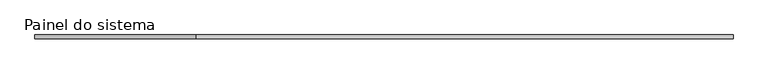
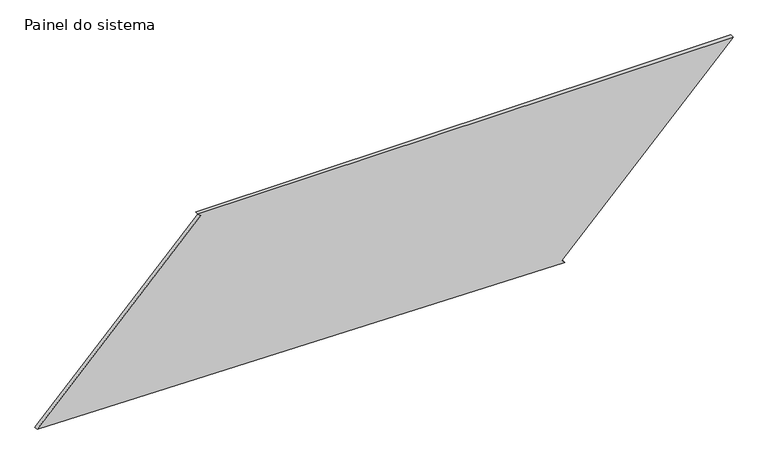
"""IFC4 building model written with IfcOpenShell, lengths in millimetres: plate geometry, Painel do sistema : Envidraçado."""

from ifc_helpers import new_model, si_unit, frame, origin, place, context, project, spatial, polyline, outline, extrude, source, transform, mapped, element, save


def painel_do_sistema_521c3f7b(model_context):
    return source(origin(), model_context, "Body", "SweptSolid", [
        extrude(outline(polyline([(0.0, 1189.455297), (17.3932625, 1171.4977243), (1188.7683803, 2306.0628062), (1188.7683803, -1240.670622), (1171.3751177, -1222.7130493), (52.8769643, -2306.0628062), (0.0, 1189.455297)])), frame((0.0, 24.5, 0.0), z_axis=(0.0, 1.0, 0.0), x_axis=(0.0, 0.0, 1.0)), (0.0, 0.0, 1.0), 25.0),
    ])


if __name__ == "__main__":
    model = new_model("IFC4")
    model_context = context("Model", 3, world=origin())
    ifc_project = project(units=[si_unit("LENGTHUNIT", "METRE", prefix="MILLI")], contexts=[model_context])
    site = spatial("IfcSite", under=ifc_project)
    building = spatial("IfcBuilding", under=site)
    placement = place(None, origin())
    painel_do_sistema_shape = painel_do_sistema_521c3f7b(model_context)
    element("IfcPlate", 1, ObjectType="Painel do sistema : Envidraçado", at=placement, inside=building, context=model_context, shape_type="MappedRepresentation", body=[
        mapped(painel_do_sistema_shape, transform((0.0, 0.0, 0.0), x_axis=(1.0, 0.0, 0.0), y_axis=(0.0, 1.0, 0.0), z_axis=(0.0, 0.0, 1.0))),
    ])
    save(model, "model.ifc")

# Revit data of these elements
# Type "Painel do sistema : Envidraçado"
#   Construction Type Id = "GSP4R"
#   Analytic Construction = "Vidraça única Pilkington 1/8 pol"
#   Visual Light Transmittance = 0.9
#   Solar Heat Gain Coefficient = 0.86
#   Heat Transfer Coefficient (U) = 6.7069 W/(m²·K)
# Element 1 (IfcPlate, "Painel do sistema : Envidraçado")
#   Materials on its faces: "Vidro"
# Materials
#   "Vidro": class "Vidro", colour RGB 0 128 192, transparency 0.9, Description = "Vidro de sílica", Cost = 0
